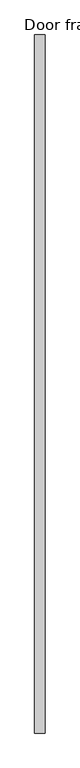
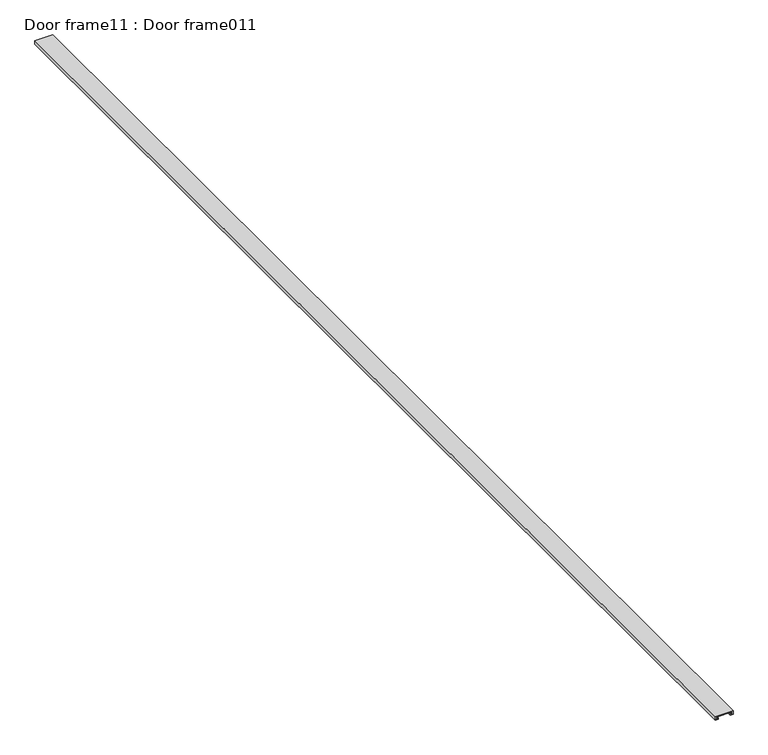
"""IFC4 building model written with IfcOpenShell, lengths in millimetres: proxy geometry, Door frame11 : Door frame011."""

import ifcopenshell
import ifcopenshell.guid

model = None  # the IFC model being written
_history = None  # IfcOwnerHistory: only IFC2X3 demands one
_inside = {}  # id of a spatial element -> (the spatial element, [elements in it])
_under = {}  # id of a project, library or spatial element -> (it, [spatial elements below it])
_declared = {}  # id of a project -> (the project, [libraries it declares])
_typed = {}  # id of a type object -> (the type object, [elements of that type])
_made_of = {}  # id of a material, layer set ... -> (it, [elements and type objects made of it])


def new_model(schema):
    """Start an empty IFC model of exactly this schema.

    Asked for "IFC4X3", IfcOpenShell would pick the latest addendum, in which some entities
    have other attributes; the version numbers below select the first issue.
    IFC2X3 requires an IfcOwnerHistory on every rooted entity: one is made here for all.
    """
    global model, _history
    if schema == "IFC4X3":
        model = ifcopenshell.file(schema_version=(4, 3, 0, 0))
    else:
        model = ifcopenshell.file(schema=schema)
    _inside.clear()
    _under.clear()
    _declared.clear()
    _typed.clear()
    _made_of.clear()
    _history = None
    if model.schema == "IFC2X3":
        org = make("IfcOrganization", Name="unknown")
        user = make(
            "IfcPersonAndOrganization",
            ThePerson=make("IfcPerson", FamilyName="unknown"),
            TheOrganization=org,
        )
        app = make(
            "IfcApplication",
            ApplicationDeveloper=org,
            Version="unknown",
            ApplicationFullName="unknown",
            ApplicationIdentifier="unknown",
        )
        _history = make(
            "IfcOwnerHistory",
            OwningUser=user,
            OwningApplication=app,
            ChangeAction="ADDED",
            CreationDate=0,
        )
    return model


def make(cls, **values):
    """One entity of the class cls with the attributes given. An attribute that is None is left unset."""
    return model.create_entity(
        cls, **{name: value for name, value in values.items() if value is not None}
    )


def rooted(cls, **values):
    """An entity with a GlobalId (a new one), such as an element, a storey or a relation."""
    return make(cls, GlobalId=ifcopenshell.guid.new(), OwnerHistory=_history, **values)


def si_unit(unit_type, name, prefix=None):
    """IfcSIUnit, for example si_unit("LENGTHUNIT", "METRE", prefix="MILLI")."""
    return make("IfcSIUnit", UnitType=unit_type, Prefix=prefix, Name=name)


def assignment(units):
    """IfcUnitAssignment: the units of a project."""
    return None if units is None else make("IfcUnitAssignment", Units=units)


def point(xyz):
    """IfcCartesianPoint."""
    return None if xyz is None else make("IfcCartesianPoint", Coordinates=xyz)


def direction(xyz):
    """IfcDirection."""
    return None if xyz is None else make("IfcDirection", DirectionRatios=xyz)


def frame(location, z_axis=None, x_axis=None):
    """IfcAxis2Placement3D, a coordinate frame: its origin and axes. An axis left out is left unset."""
    return make(
        "IfcAxis2Placement3D",
        Location=point(location),
        Axis=direction(z_axis),
        RefDirection=direction(x_axis),
    )


def origin():
    """The frame at (0, 0, 0) with its axes left unset."""
    return frame((0.0, 0.0, 0.0))


def place(relative_to, where):
    """IfcLocalPlacement: puts the frame where relative to a parent placement (None: the world)."""
    return make(
        "IfcLocalPlacement", PlacementRelTo=relative_to, RelativePlacement=where
    )


def context(
    kind, dimensions, precision=None, world=None, true_north=None, identifier=None
):
    """IfcGeometricRepresentationContext, for example the 3D "Model" context."""
    return make(
        "IfcGeometricRepresentationContext",
        ContextIdentifier=identifier,
        ContextType=kind,
        CoordinateSpaceDimension=dimensions,
        Precision=precision,
        WorldCoordinateSystem=world,
        TrueNorth=true_north,
    )


def project(units=None, contexts=None):
    """IfcProject with its units and contexts."""
    return rooted(
        "IfcProject",
        Name="project",
        RepresentationContexts=contexts,
        UnitsInContext=assignment(units),
    )


def spatial(cls, under=None, at=None, **own):
    """A site, building, storey or space (cls), placed at a placement, below another one or the project."""
    s = rooted(cls, ObjectPlacement=at, **own)
    if under is not None:
        _under.setdefault(under.id(), (under, []))[1].append(s)
    return s


def polyline(points):
    """IfcPolyline through the points."""
    return make("IfcPolyline", Points=[point(p) for p in points])


def outline(outer, holes=None, kind="AREA"):
    """IfcArbitraryClosedProfileDef: a profile drawn as a closed curve; with holes, ...WithVoids."""
    if holes is None:
        return make("IfcArbitraryClosedProfileDef", ProfileType=kind, OuterCurve=outer)
    return make(
        "IfcArbitraryProfileDefWithVoids",
        ProfileType=kind,
        OuterCurve=outer,
        InnerCurves=holes,
    )


def extrude(swept, where, along, depth):
    """IfcExtrudedAreaSolid: the profile swept, set in the frame where, extruded along a direction by depth."""
    return make(
        "IfcExtrudedAreaSolid",
        SweptArea=swept,
        Position=where,
        ExtrudedDirection=direction(along),
        Depth=depth,
    )


def shape(context_of_items, identifier, shape_type, items):
    """IfcShapeRepresentation: the items that make up one representation, for example the "Body"."""
    return make(
        "IfcShapeRepresentation",
        ContextOfItems=context_of_items,
        RepresentationIdentifier=identifier,
        RepresentationType=shape_type,
        Items=items,
    )


def source(mapping_origin, context_of_items, identifier, shape_type, items):
    """IfcRepresentationMap: a shape defined once, which mapped items show again and again."""
    return make(
        "IfcRepresentationMap",
        MappingOrigin=mapping_origin,
        MappedRepresentation=shape(context_of_items, identifier, shape_type, items),
    )


def transform(
    local_origin,
    x_axis=None,
    y_axis=None,
    z_axis=None,
    scale=None,
    scale2=None,
    scale3=None,
    uniform=True,
):
    """IfcCartesianTransformationOperator3D, or its non-uniform kind. x_axis, y_axis, z_axis: its Axis1, 2, 3."""
    if uniform:
        return make(
            "IfcCartesianTransformationOperator3D",
            Axis1=direction(x_axis),
            Axis2=direction(y_axis),
            LocalOrigin=point(local_origin),
            Scale=scale,
            Axis3=direction(z_axis),
        )
    return make(
        "IfcCartesianTransformationOperator3DnonUniform",
        Axis1=direction(x_axis),
        Axis2=direction(y_axis),
        LocalOrigin=point(local_origin),
        Scale=scale,
        Axis3=direction(z_axis),
        Scale2=scale2,
        Scale3=scale3,
    )


def mapped(mapping_source, mapping_target):
    """IfcMappedItem: shows the shape of a source again, moved by a transform."""
    return make(
        "IfcMappedItem", MappingSource=mapping_source, MappingTarget=mapping_target
    )


def made_of(thing, what):
    """Note that an element or type object is made of a material, layer set ...; save() writes the relation."""
    if what is not None:
        _made_of.setdefault(what.id(), (what, []))[1].append(thing)
    return thing


def element(
    cls,
    number,
    at=None,
    inside=None,
    cuts=None,
    type_object=None,
    material=None,
    context=None,
    identifier="Body",
    shape_type=None,
    held_by="IfcProductDefinitionShape",
    body=None,
    shapes=None,
    **own,
):
    """One element of the class cls, such as IfcWall. Its Tag is "e" and its number.

    at: its placement. inside: the storey or other place that contains it. cuts: it is an
    opening in that element (IfcRelVoidsElement). A single representation is given by context,
    identifier, shape_type and body (its items); several are given by shapes. held_by: the class
    of the entity that holds the representations. save() writes the other relations.
    """
    e = rooted(cls, Tag="e%d" % number, ObjectPlacement=at, **own)
    if body is not None:
        shapes = [shape(context, identifier, shape_type, body)]
    if shapes is not None:
        e.Representation = make(held_by, Representations=shapes)
    if inside is not None:
        _inside.setdefault(inside.id(), (inside, []))[1].append(e)
    if cuts is not None:
        rooted(
            "IfcRelVoidsElement", RelatingBuildingElement=cuts, RelatedOpeningElement=e
        )
    if type_object is not None:
        _typed.setdefault(type_object.id(), (type_object, []))[1].append(e)
    return made_of(e, material)


def aggregate(whole, parts):
    """IfcRelAggregates: a whole, such as a stair, and the parts it consists of."""
    return rooted("IfcRelAggregates", RelatingObject=whole, RelatedObjects=parts)


def save(model, path):
    """Write the relations noted so far, then the file.

    IfcRelAggregates (storeys below a building ...), IfcRelContainedInSpatialStructure (elements
    in a storey), IfcRelDefinesByType, IfcRelAssociatesMaterial and IfcRelDeclares: one each for
    every whole, place, type object, material and project.
    """
    for whole, parts in _under.values():
        aggregate(whole, parts)
    for where, things in _inside.values():
        rooted(
            "IfcRelContainedInSpatialStructure",
            RelatedElements=things,
            RelatingStructure=where,
        )
    for kind, things in _typed.values():
        rooted("IfcRelDefinesByType", RelatedObjects=things, RelatingType=kind)
    for what, things in _made_of.values():
        rooted("IfcRelAssociatesMaterial", RelatedObjects=things, RelatingMaterial=what)
    for by, libraries in _declared.values():
        rooted("IfcRelDeclares", RelatingContext=by, RelatedDefinitions=libraries)
    model.write(path)


def door_frame11_door_frame011_5bdfa61c(model_context):
    return source(origin(), model_context, "Body", "SweptSolid", [
        extrude(outline(polyline([(36591.6240434, 15510.0170405), (36585.6418094, 15510.0170405), (36585.6418094, 15514.9588645), (36588.2201312, 15514.9588645), (36588.2201312, 15513.9184805), (36586.9422894, 15513.9184805), (36586.9422894, 15511.3174945), (36590.0634674, 15511.3174945), (36590.0634674, 15538.9397417), (36586.9422894, 15538.9397417), (36586.9422894, 15536.538273), (36588.2201312, 15536.538273), (36588.2201312, 15535.2983717), (36585.6418094, 15535.2983717), (36585.6418094, 15540.2401957), (36591.6240434, 15540.2401957), (36591.6240434, 15510.0170405)])), frame((0.0, -1052.8906567, 0.0), z_axis=(0.0, 1.0, 0.0), x_axis=(0.0, 0.0, 1.0)), (0.0, 0.0, 1.0), 1999.85),
    ])


if __name__ == "__main__":
    model = new_model("IFC4")
    model_context = context("Model", 3, world=origin())
    ifc_project = project(units=[si_unit("LENGTHUNIT", "METRE", prefix="MILLI")], contexts=[model_context])
    site = spatial("IfcSite", under=ifc_project)
    building = spatial("IfcBuilding", under=site)
    placement = place(None, origin())
    door_frame11_door_frame011_shape = door_frame11_door_frame011_5bdfa61c(model_context)
    element("IfcBuildingElementProxy", 1, Name="Door frame11 : Door frame011", ObjectType="Door frame11 : Door frame011", at=placement, inside=building, context=model_context, shape_type="MappedRepresentation", body=[
        mapped(door_frame11_door_frame011_shape, transform((0.0, 0.0, 0.0), x_axis=(1.0, 0.0, 0.0), y_axis=(0.0, 1.0, 0.0), z_axis=(0.0, 0.0, 1.0))),
    ])
    save(model, "model.ifc")

# Revit data of these elements
# Type "Door frame11 : Door frame011"
#   NameOverride = "Door frame011"
# Element 1 (IfcBuildingElementProxy, "Door frame11 : Door frame011")
#   Materials on its faces: "FLEETWOOD SERIES T-3200 SINGLE SWING DOOR FRAME"
# Materials
#   "FLEETWOOD SERIES T-3200 SINGLE SWING DOOR FRAME": class "Unassigned", colour RGB 128 128 128, transparency 0, Cost = 0
